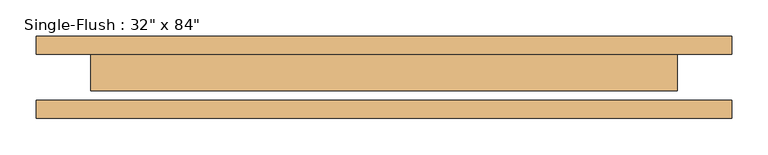
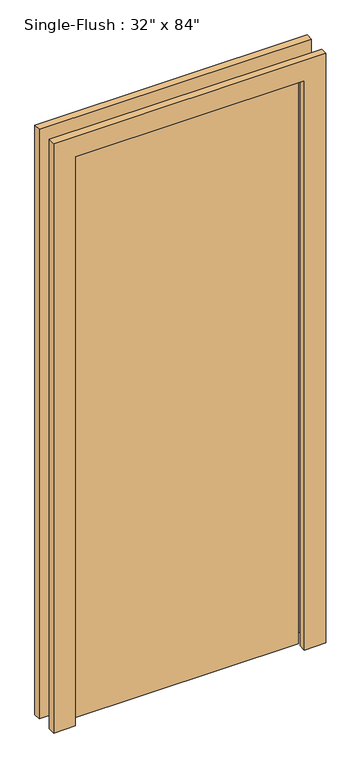
"""IFC4 building model written with IfcOpenShell, lengths in millimetres: door geometry."""

from ifc_helpers import new_model, si_unit, frame, origin, origin_with_axes, place, context, project, spatial, polyline, outline, extrude, source, transform, mapped, element, save


def door_6e402fa7(model_context):
    return source(origin(), model_context, "Body", "SweptSolid", [
        extrude(outline(polyline([(2209.8, -482.6), (0.0, -482.6), (0.0, -406.4), (2133.6, -406.4), (2133.6, 406.4), (0.0, 406.4), (0.0, 482.6), (2209.8, 482.6), (2209.8, -482.6)])), frame((0.0, 31.75, 0.0), z_axis=(0.0, 1.0, 0.0), x_axis=(0.0, 0.0, 1.0)), (0.0, 0.0, 1.0), 25.4),
        extrude(outline(polyline([(2209.8, 482.6), (2209.8, -482.6), (0.0, -482.6), (0.0, -406.4), (2133.6, -406.4), (2133.6, 406.4), (0.0, 406.4), (0.0, 482.6), (2209.8, 482.6)])), frame((0.0, -57.15, 0.0), z_axis=(0.0, 1.0, 0.0), x_axis=(0.0, 0.0, 1.0)), (0.0, 0.0, 1.0), 25.4),
        extrude(outline(polyline([(406.4, -19.05), (-406.4, -19.05), (-406.4, 31.75), (406.4, 31.75), (406.4, -19.05)])), origin_with_axes(), (0.0, 0.0, 1.0), 2133.6),
    ])


if __name__ == "__main__":
    model = new_model("IFC4")
    model_context = context("Model", 3, world=origin())
    ifc_project = project(units=[si_unit("LENGTHUNIT", "METRE", prefix="MILLI")], contexts=[model_context])
    site = spatial("IfcSite", under=ifc_project)
    building = spatial("IfcBuilding", under=site)
    placement = place(None, origin())
    door_shape = door_6e402fa7(model_context)
    element("IfcDoor", 1, ObjectType="Single-Flush : 32\" x 84\"", at=placement, inside=building, context=model_context, shape_type="MappedRepresentation", body=[
        mapped(door_shape, transform((0.0, 0.0, 0.0), x_axis=(1.0, 0.0, 0.0), y_axis=(0.0, 1.0, 0.0), z_axis=(0.0, 0.0, 1.0))),
    ])
    save(model, "model.ifc")

# Revit data of these elements
# Type "Single-Flush : 32\" x 84\""
#   Type Mark = "3"
#   Construction Type Id = "MDOOR"
#   Assembly Code = "C1020"
#   Analytic Construction = "Metal"
#   Thickness = 0' - 2"
#   Heat Transfer Coefficient (U) = 0.651978 BTU/(h·ft²·°F)
#   Height = 7' - 0"
#   Trim Projection Ext = 0' - 1"
#   Trim Projection Int = 0' - 1"
#   Trim Width = 0' - 3"
#   Width = 2' - 8"
#   Define Thermal Properties by = 1
#   Define Thermal Properties by = 1
#   Door Material = Door - Panel
#   Frame Material = Door - Frame
#   Visual Light Transmittance = 0
#   Solar Heat Gain Coefficient = 0
#   Function = (empty or 0)
#   Wall Closure = (empty or 0)
# Element 1 (IfcDoor, "Single-Flush : 32\" x 84\"")
#   Materials on its faces: "Door - Frame", "Door - Panel"
# Materials
#   "Door - Panel": class "Wood", colour RGB 210 159 95, transparency 0, Cost = 0
#   "Door - Frame": class "Miscellaneous", colour RGB 118 70 51, transparency 0, Cost = 0
